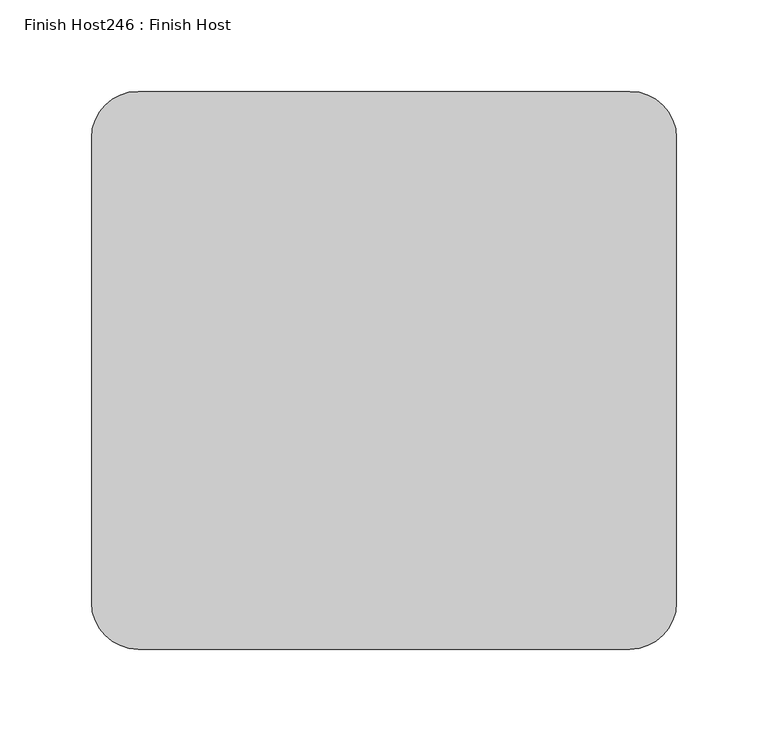
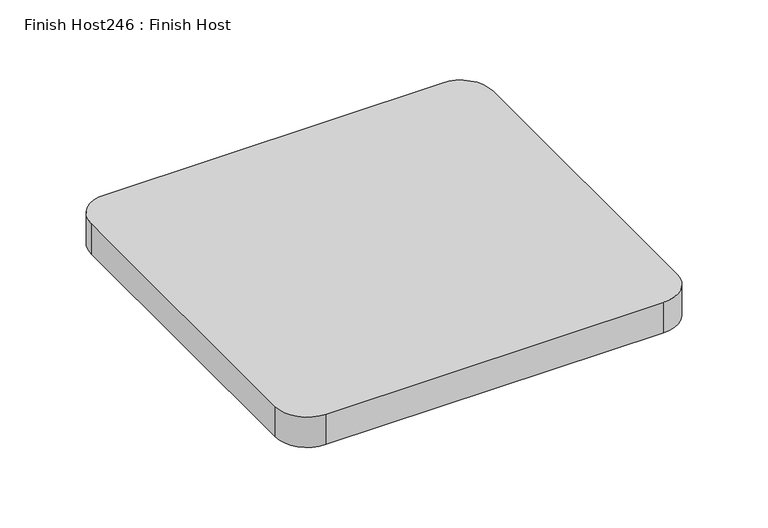
"""IFC4 building model written with IfcOpenShell, lengths in millimetres: proxy geometry, Finish Host246 : Finish Host."""

from ifc_helpers import new_model, si_unit, point, frame_2d, origin, origin_with_axes, place, context, project, spatial, polyline, circle_curve, trimmed, segment, composite_curve, outline, extrude, source, transform, mapped, element, save


def finish_host246_finish_host_0a5a82de(model_context):
    return source(origin(), model_context, "Body", "SweptSolid", [
        extrude(outline(composite_curve([segment(polyline([(-49.9083644, 3462.3960864), (-49.9083644, 3716.3960864)]), True, "CONTINUOUS"), segment(trimmed(circle_curve(frame_2d((-24.5083644, 3716.3960864)), 25.4), [point((-49.9083644, 3716.3960864))], [point((-24.5083644, 3741.7960864))], False, "CARTESIAN"), True, "CONTINUOUS"), segment(polyline([(-24.5083644, 3741.7960864), (244.2157184, 3741.7960864)]), True, "CONTINUOUS"), segment(trimmed(circle_curve(frame_2d((244.2157184, 3716.3960864)), 25.4), [point((244.2157184, 3741.7960864))], [point((269.6157184, 3716.3960864))], False, "CARTESIAN"), True, "CONTINUOUS"), segment(polyline([(269.6157184, 3716.3960864), (269.6157184, 3462.3960864)]), True, "CONTINUOUS"), segment(trimmed(circle_curve(frame_2d((244.2157184, 3462.3960864)), 25.4), [point((269.6157184, 3462.3960864))], [point((244.2157184, 3436.9960864))], False, "CARTESIAN"), True, "CONTINUOUS"), segment(polyline([(244.2157184, 3436.9960864), (-24.5083644, 3436.9960864)]), True, "CONTINUOUS"), segment(trimmed(circle_curve(frame_2d((-24.5083644, 3462.3960864)), 25.4), [point((-24.5083644, 3436.9960864))], [point((-49.9083644, 3462.3960864))], False, "CARTESIAN"), True, "CONTINUOUS")], self_intersect=False)), origin_with_axes(), (0.0, 0.0, 1.0), 25.4),
    ])


if __name__ == "__main__":
    model = new_model("IFC4")
    model_context = context("Model", 3, world=origin())
    ifc_project = project(units=[si_unit("LENGTHUNIT", "METRE", prefix="MILLI")], contexts=[model_context])
    site = spatial("IfcSite", under=ifc_project)
    building = spatial("IfcBuilding", under=site)
    placement = place(None, origin())
    finish_host246_finish_host_shape = finish_host246_finish_host_0a5a82de(model_context)
    element("IfcBuildingElementProxy", 1, Name="Finish Host246 : Finish Host", ObjectType="Finish Host246 : Finish Host", at=placement, inside=building, context=model_context, shape_type="MappedRepresentation", body=[
        mapped(finish_host246_finish_host_shape, transform((0.0, 0.0, 0.0), x_axis=(1.0, 0.0, 0.0), y_axis=(0.0, 1.0, 0.0), z_axis=(0.0, 0.0, 1.0))),
    ])
    save(model, "model.ifc")

# Revit data of these elements
# Project information
#   Project Issue Date = "Issue Date"
#   Project Status = "Project Status"
#   Client Name = "Owner"
#   Project Address = "Enter address here"
#   Project Name = "Project Name"
#   Project Number = "Project Number"
# Type "Finish Host246 : Finish Host"
#   Countertop Material = Fabric - Teknion - E386 - Essentials - Forsythia
# Element 1 (IfcBuildingElementProxy, "Finish Host246 : Finish Host")
#   Materials on its faces: "Fabric - Teknion - E386 - Essentials - Forsythia"
# Materials
#   "Fabric - Teknion - E386 - Essentials - Forsythia": class "Fabric", colour RGB 68 61 42, transparency 0, Model = "E386", Manufacturer = "Teknion Studio", URL = "http://www.teknionstudio.com/", Description = "Forsytia Essentials", Cost = 0
